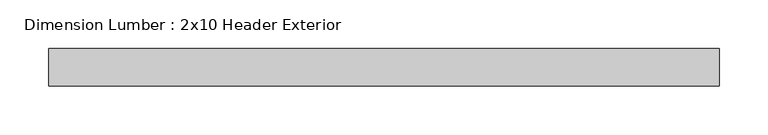
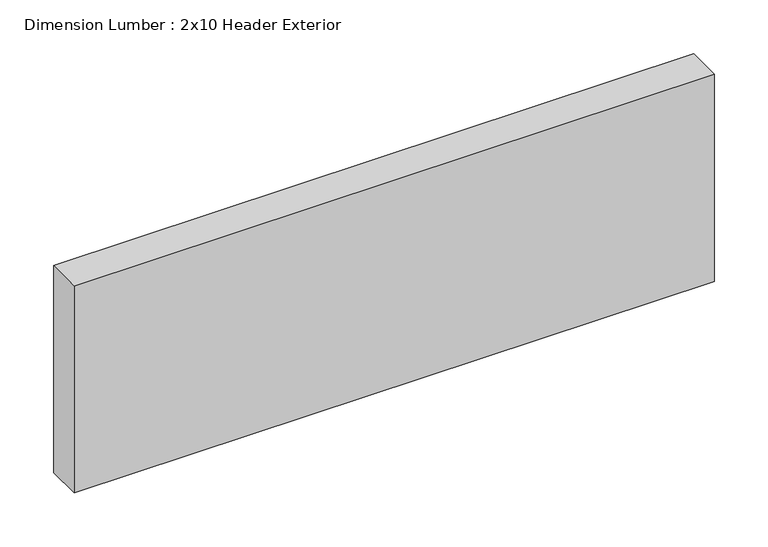
"""IFC4 building model written with IfcOpenShell, lengths in millimetres: beam geometry, Dimension Lumber : 2x10 Header Exterior."""

from ifc_helpers import new_model, si_unit, frame, origin, place, context, project, spatial, polyline, outline, extrude, source, transform, mapped, element, save


def dimension_lumber_2x10_header_exterior_0c196d91(model_context):
    return source(origin(), model_context, "Body", "SweptSolid", [
        extrude(outline(polyline([(468.709375, 19.05), (468.709375, -19.05), (-217.090625, -19.05), (-217.090625, 19.05), (468.709375, 19.05)])), frame((0.0, 0.0, -117.475), z_axis=(0.0, 0.0, 1.0), x_axis=(1.0, 0.0, 0.0)), (0.0, 0.0, 1.0), 234.95),
    ])


if __name__ == "__main__":
    model = new_model("IFC4")
    model_context = context("Model", 3, world=origin())
    ifc_project = project(units=[si_unit("LENGTHUNIT", "METRE", prefix="MILLI")], contexts=[model_context])
    site = spatial("IfcSite", under=ifc_project)
    building = spatial("IfcBuilding", under=site)
    placement = place(None, origin())
    dimension_lumber_2x10_header_exterior_shape = dimension_lumber_2x10_header_exterior_0c196d91(model_context)
    element("IfcBeam", 1, ObjectType="Dimension Lumber : 2x10 Header Exterior", at=placement, inside=building, context=model_context, shape_type="MappedRepresentation", body=[
        mapped(dimension_lumber_2x10_header_exterior_shape, transform((0.0, 0.0, 0.0), x_axis=(1.0, 0.0, 0.0), y_axis=(0.0, 1.0, 0.0), z_axis=(0.0, 0.0, 1.0))),
    ])
    save(model, "model.ifc")

# Revit data of these elements
# Type "Dimension Lumber : 2x10 Header Exterior"
#   Assembly Code = "B10"
#   A = 0.0963889 SF
#   Length [instance default] = 5' - 0"
#   b = 0' - 1 1/2"
#   d = 0' - 9 1/4"
#   Structural Material [instance default] = Softwood, Lumber
# Element 1 (IfcBeam, "Dimension Lumber : 2x10 Header Exterior")
#   Structural Material = Douglas Fir #2
#   Materials on its faces: "Douglas Fir #2"
# Materials
#   "Softwood, Lumber": class "Wood", colour RGB 223 192 134, transparency 0, Description = "Pinus Echinata", Cost = 0
#   "Douglas Fir #2": class "Wood", colour RGB 223 192 134, transparency 0, Description = "Pinus Echinata", Cost = 0
